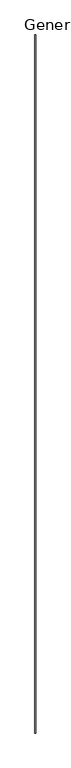
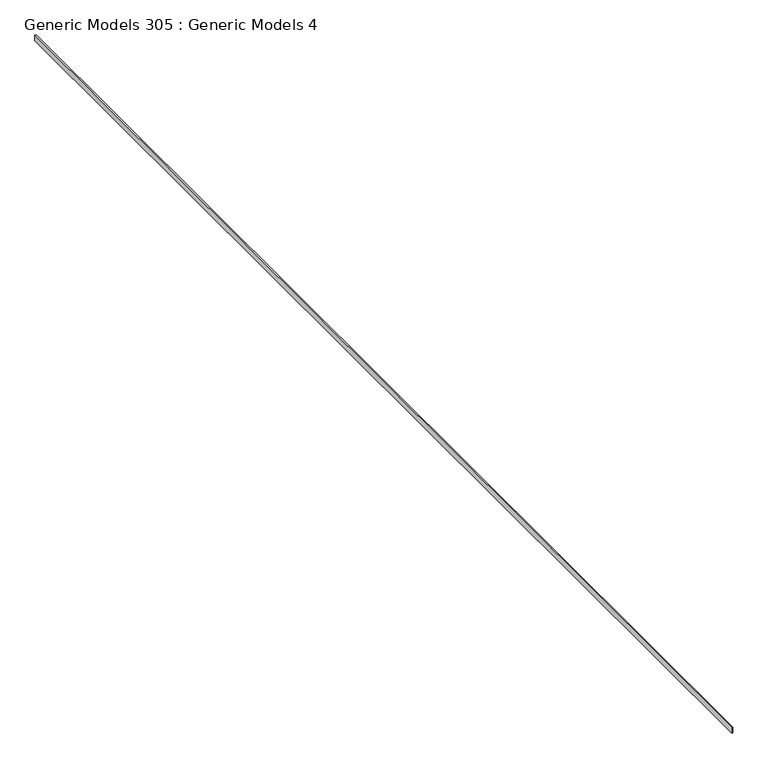
"""IFC4 building model written with IfcOpenShell, lengths in millimetres: proxy geometry, Generic Models 305 : Generic Models 4."""

from ifc_helpers import new_model, si_unit, frame, origin, place, context, project, spatial, polyline, outline, extrude, source, transform, mapped, element, save


def generic_models_305_generic_models_4_707eb8d8(model_context):
    return source(origin(), model_context, "Body", "SweptSolid", [
        extrude(outline(polyline([(-6912.0940869, -5493.3230338), (-6924.7940869, -5493.3230338), (-6924.7940869, 7054.2769662), (-6912.0940869, 7054.2769662), (-6912.0940869, -5493.3230338)])), frame((0.0, 0.0, 123069.096), z_axis=(0.0, 0.0, 1.0), x_axis=(1.0, 0.0, 0.0)), (0.0, 0.0, 1.0), 62.1422763),
    ])


if __name__ == "__main__":
    model = new_model("IFC4")
    model_context = context("Model", 3, world=origin())
    ifc_project = project(units=[si_unit("LENGTHUNIT", "METRE", prefix="MILLI")], contexts=[model_context])
    site = spatial("IfcSite", under=ifc_project)
    building = spatial("IfcBuilding", under=site)
    placement = place(None, origin())
    generic_models_305_generic_models_4_shape = generic_models_305_generic_models_4_707eb8d8(model_context)
    element("IfcBuildingElementProxy", 1, Name="Generic Models 305 : Generic Models 4", ObjectType="Generic Models 305 : Generic Models 4", at=placement, inside=building, context=model_context, shape_type="MappedRepresentation", body=[
        mapped(generic_models_305_generic_models_4_shape, transform((0.0, 0.0, 0.0), x_axis=(1.0, 0.0, 0.0), y_axis=(0.0, 1.0, 0.0), z_axis=(0.0, 0.0, 1.0))),
    ])
    save(model, "model.ifc")

# Revit data of these elements
# Element 1 (IfcBuildingElementProxy, "Generic Models 305 : Generic Models 4")
#   Materials on its faces: "_CONCRETE EXPANSION JOINT - MINERAL FIBER"
# Materials
#   "_CONCRETE EXPANSION JOINT - MINERAL FIBER": class "Generic", colour RGB 190 220 196, transparency 0, Cost = 0
